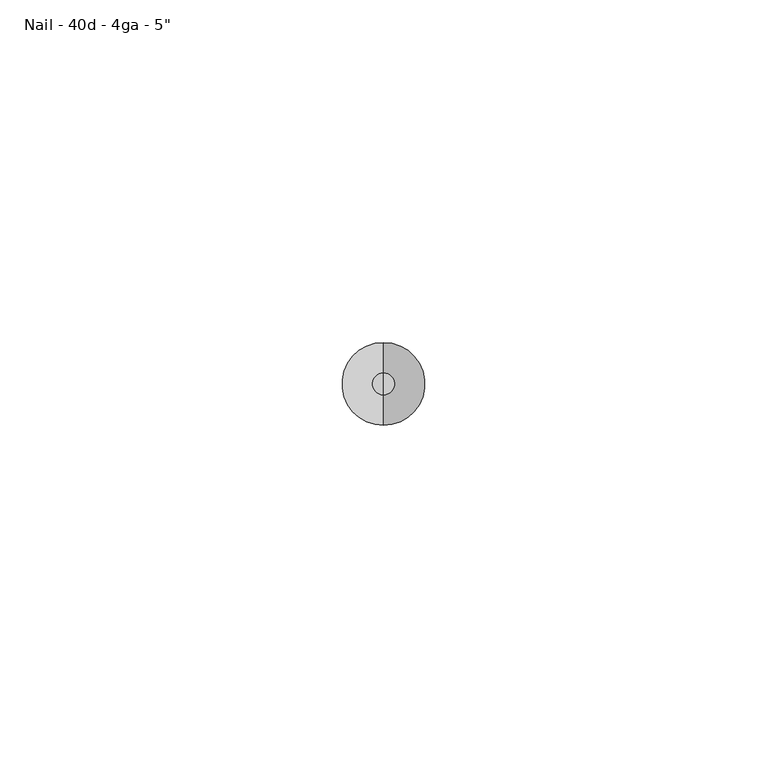
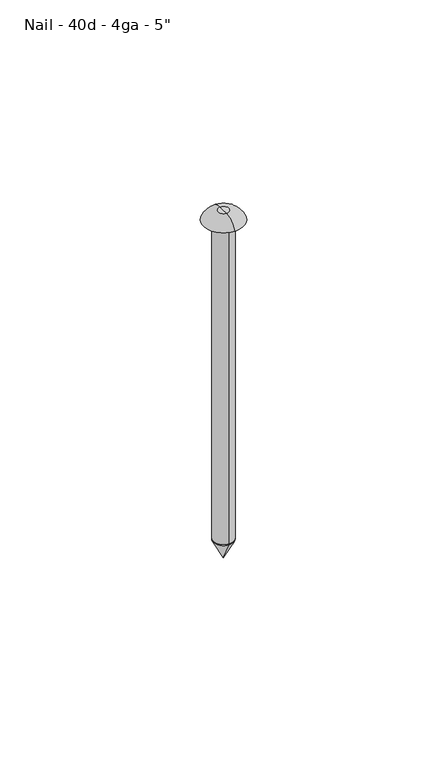
"""IFC4 building model written with IfcOpenShell, lengths in millimetres: fastener geometry."""

from ifc_helpers import new_model, si_unit, point, frame, origin, origin_2d, place, context, project, spatial, polyline, circle_curve, ellipse_curve, trimmed, segment, composite_curve, outline, extrude, source, transform, mapped, element, save
from ifc_brep_helpers import plane_surface, revolved_surface, advanced_brep


def fastener_0606e984(model_context):
    return source(origin(), model_context, "Body", "SolidModel", [
        advanced_brep(
        [(0.0, -3.0226, -101.6), (0.0, 3.0226, -101.6), (0.0, 0.0, -101.6), (0.0, 0.0, -107.6452)],
        [
            (0, 1, circle_curve(frame((0.0, 0.0, -101.6), z_axis=(0.0, 0.0, 1.0), x_axis=(0.0, 1.0, 0.0)), 3.0226)),
            (1, 2),
            (2, 0),
            (1, 0, circle_curve(frame((0.0, 0.0, -101.6), z_axis=(0.0, 0.0, 1.0), x_axis=(0.0, 1.0, 0.0)), 3.0226)),
            (3, 1),
            (0, 3),
        ],
        [
            plane_surface(frame((0.0, 0.0, -101.6), z_axis=(0.0, 0.0, 1.0), x_axis=(0.0, 1.0, 0.0))),
            revolved_surface(polyline([(0.0, 3.0226, -101.6), (0.0, 0.0, -107.6452)]), (0.0, 0.0, -103.0840259), (0.0, 0.0, -1.0)),
        ],
        [
            (0, [[1, 2, 3]]),
            (0, [[4, -3, -2]]),
            (1, [[5, -1, 6]]),
            (1, [[-6, -4, -5]]),
        ],
    ),
        advanced_brep(
        [(0.0, 6.0452, 0.0), (0.0, -6.0452, 0.0), (0.0, 0.0, 0.0), (0.0, 0.0, 3.0226), (0.0, -1.5875, 3.0226), (0.0, 1.5875, 3.0226)],
        [
            (0, 1, circle_curve(frame((0.0, 0.0, 0.0), z_axis=(0.0, 0.0, -1.0), x_axis=(0.0, -1.0, 0.0)), 6.0452)),
            (1, 2),
            (2, 0),
            (1, 0, circle_curve(frame((0.0, 0.0, 0.0), z_axis=(0.0, 0.0, -1.0), x_axis=(0.0, -1.0, 0.0)), 6.0452)),
            (3, 4),
            (4, 5, circle_curve(frame((0.0, 0.0, 3.0226), z_axis=(0.0, 0.0, 1.0), x_axis=(0.0, -1.0, 0.0)), 1.5875)),
            (5, 3),
            (5, 4, circle_curve(frame((0.0, 0.0, 3.0226), z_axis=(0.0, 0.0, 1.0), x_axis=(0.0, -1.0, 0.0)), 1.5875)),
            (4, 1, circle_curve(frame((0.0, -1.5875, -1.7757855), z_axis=(1.0, 0.0, 0.0), x_axis=(0.0, -1.0, 0.0)), 4.7983855)),
            (0, 5, circle_curve(frame((0.0, 1.5875, -1.7757855), z_axis=(1.0, 0.0, 0.0), x_axis=(0.0, 1.0, 0.0)), 4.7983855)),
        ],
        [
            plane_surface(frame((0.0, 0.0, 0.0), z_axis=(0.0, 0.0, -1.0), x_axis=(0.0, -1.0, 0.0))),
            plane_surface(frame((0.0, 0.0, 3.0226), z_axis=(0.0, 0.0, 1.0), x_axis=(0.0, -1.0, 0.0))),
            revolved_surface(trimmed(ellipse_curve(frame((0.0, -1.5875, -1.7757855), z_axis=(-1.0, 0.0, 0.0), x_axis=(0.0, -1.0, 0.0)), 4.7983855, 4.7983855), [point((0.0, -6.0452, 0.0))], [point((0.0, -1.5875, 3.0226))], True, "CARTESIAN"), (0.0, 0.0, 1.4840259), (0.0, 0.0, 1.0)),
        ],
        [
            (0, [[1, 2, 3]]),
            (0, [[4, -3, -2]]),
            (1, [[5, 6, 7]]),
            (1, [[-7, 8, -5]]),
            (2, [[-6, 9, -1, 10]]),
            (2, [[-8, -10, -4, -9]]),
        ],
    ),
        extrude(outline(composite_curve([segment(trimmed(circle_curve(origin_2d(), 3.0226), [point((0.0, -3.0226))], [point((0.0, 3.0226))], False, "CARTESIAN"), True, "CONTINUOUS"), segment(trimmed(circle_curve(origin_2d(), 3.0226), [point((0.0, 3.0226))], [point((0.0, -3.0226))], False, "CARTESIAN"), True, "CONTINUOUS")], self_intersect=False)), frame((0.0, 0.0, -101.6), z_axis=(0.0, 0.0, 1.0), x_axis=(1.0, 0.0, 0.0)), (0.0, 0.0, 1.0), 101.6),
    ])


if __name__ == "__main__":
    model = new_model("IFC4")
    model_context = context("Model", 3, world=origin())
    ifc_project = project(units=[si_unit("LENGTHUNIT", "METRE", prefix="MILLI")], contexts=[model_context])
    site = spatial("IfcSite", under=ifc_project)
    building = spatial("IfcBuilding", under=site)
    placement = place(None, origin())
    fastener_shape = fastener_0606e984(model_context)
    element("IfcFastener", 1, ObjectType="060523 - W_P_C - Fastenings - Generic : Nail - 40d - 4ga - 5\"", at=placement, inside=building, context=model_context, shape_type="MappedRepresentation", body=[
        mapped(fastener_shape, transform((0.0, 0.0, 0.0), x_axis=(1.0, 0.0, 0.0), y_axis=(0.0, 1.0, 0.0), z_axis=(0.0, 0.0, 1.0))),
    ])
    save(model, "model.ifc")

# Revit data of these elements
# Type "060523 - W_P_C - Fastenings - Generic : Nail - 40d - 4ga - 5\""
#   Washer_Thickness = 0' - 0.00333"
#   Washer Radius = 0' - 0.129"
#   Washer Offset - Head = 0' - 0"
#   Washer Offset = 0' - 0"
#   Thickness_of_Substrate [instance default] = 0' - 1"
#   Side = 0' - 0 37/64"
#   Radius = 0' - 0.119"
#   Length [instance default] = 0' - 5"
#   Head Size = 0' - 1"
#   Head Radius = 0' - 0 1/2"
#   Head Height = 0' - 0.01"
#   Double Diameter = 0' - 0.476"
#   Diameter = 0' - 0.238"
#   Default Elevation = 4' - 0"
#   Washer_Nut_Visibility = no
#   Washer_Head_Visibility = no
#   Round_Head_Visibility = yes
#   Point Visibility = yes
#   Nut_Visibility = no
#   Hex_Head_Visiblilty = no
#   Washer Material = none
#   Bolt Material (Size) = AT SILL - FASTENER AT 24" O.C.
# Element 1 (IfcFastener, "060523 - W_P_C - Fastenings - Generic : Nail - 40d - 4ga - 5\"")
#   Length = 0' - 4"
#   Materials on its faces: "AT SILL - FASTENER AT 24\" O.C."
# Materials
#   "AT SILL - FASTENER AT 24\" O.C.": class "Generic", colour RGB 120 120 120, transparency 0, Cost = 0
